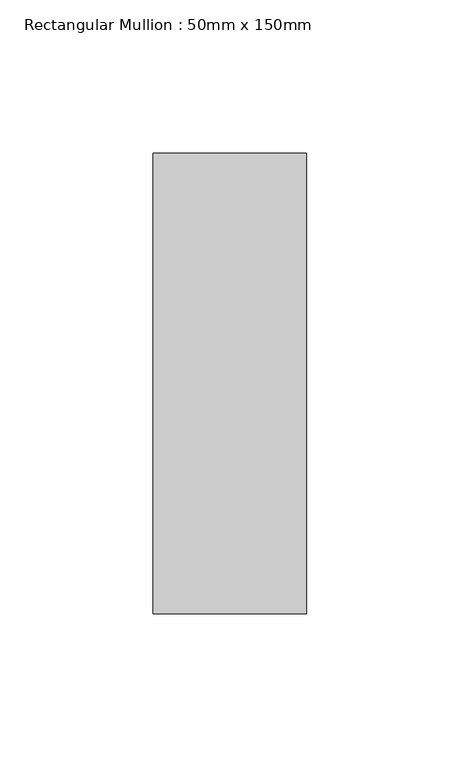
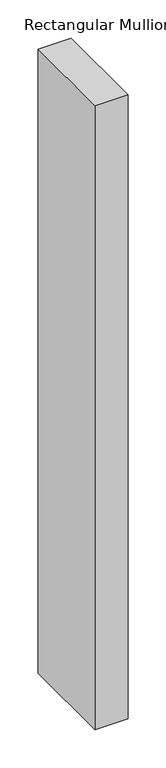
"""IFC4 building model written with IfcOpenShell, lengths in millimetres: member geometry, Rectangular Mullion : 50mm x 150mm."""

from ifc_helpers import new_model, si_unit, frame, origin, place, context, project, spatial, polyline, outline, extrude, source, transform, mapped, element, save


def rectangular_mullion_50mm_x_150mm_eeb88b28(model_context):
    return source(origin(), model_context, "Body", "SweptSolid", [
        extrude(outline(polyline([(0.0, 75.0), (0.0, -75.0), (-50.0, -75.0), (-50.0, 75.0), (0.0, 75.0)])), frame((0.0, 0.0, -1000.0), z_axis=(0.0, 0.0, 1.0), x_axis=(1.0, 0.0, 0.0)), (0.0, 0.0, 1.0), 1000.0),
    ])


if __name__ == "__main__":
    model = new_model("IFC4")
    model_context = context("Model", 3, world=origin())
    ifc_project = project(units=[si_unit("LENGTHUNIT", "METRE", prefix="MILLI")], contexts=[model_context])
    site = spatial("IfcSite", under=ifc_project)
    building = spatial("IfcBuilding", under=site)
    placement = place(None, origin())
    rectangular_mullion_50mm_x_150mm_shape = rectangular_mullion_50mm_x_150mm_eeb88b28(model_context)
    element("IfcMember", 1, ObjectType="Rectangular Mullion : 50mm x 150mm", at=placement, inside=building, context=model_context, shape_type="MappedRepresentation", body=[
        mapped(rectangular_mullion_50mm_x_150mm_shape, transform((0.0, 0.0, 0.0), x_axis=(1.0, 0.0, 0.0), y_axis=(0.0, 1.0, 0.0), z_axis=(0.0, 0.0, 1.0))),
    ])
    save(model, "model.ifc")

# Revit data of these elements
# Type "Rectangular Mullion : 50mm x 150mm"
#   built-in parameter 1007304 = 0.492126 (stored number, unit not read)
#   built-in parameter 1007301 = 0.082021 (stored number, unit not read)
#   built-in parameter 1007300 = 0.082021 (stored number, unit not read)
# Element 1 (IfcMember, "Rectangular Mullion : 50mm x 150mm")
#   Materials on its faces: "Aluminum"
# Materials
#   "Aluminum": class "Metal", colour RGB 244 244 244, transparency 0, Description = "Aluminum 6061", Cost = 0
